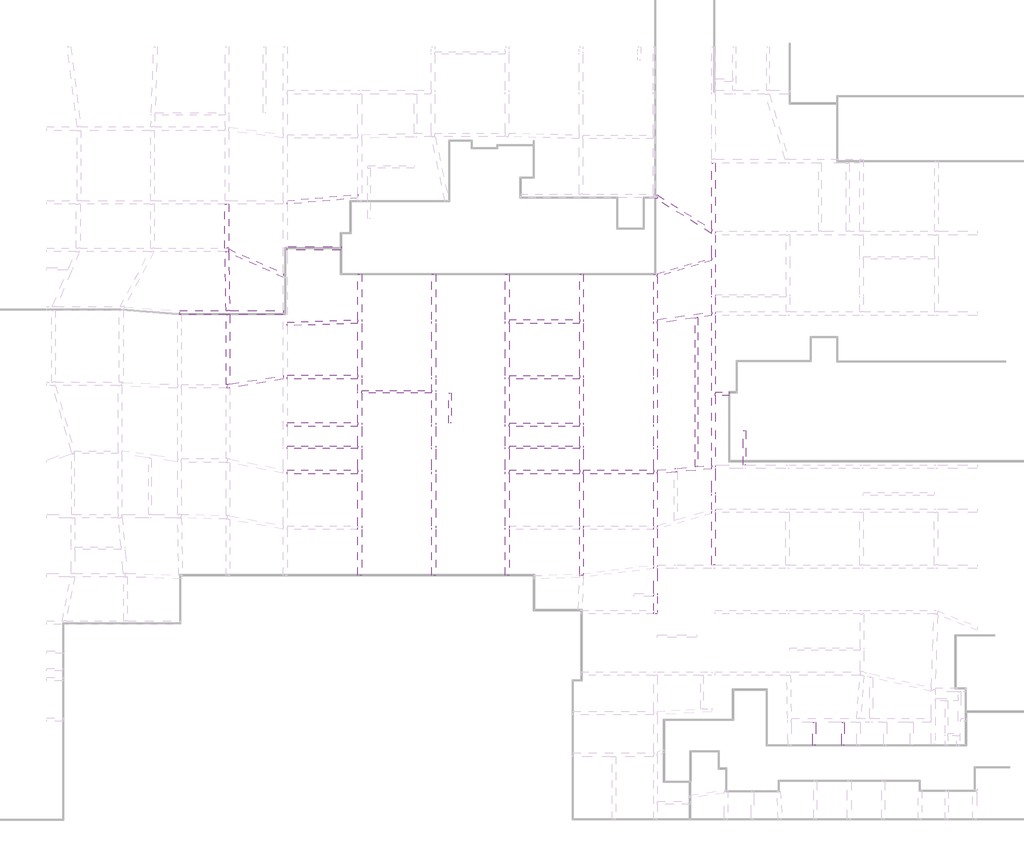
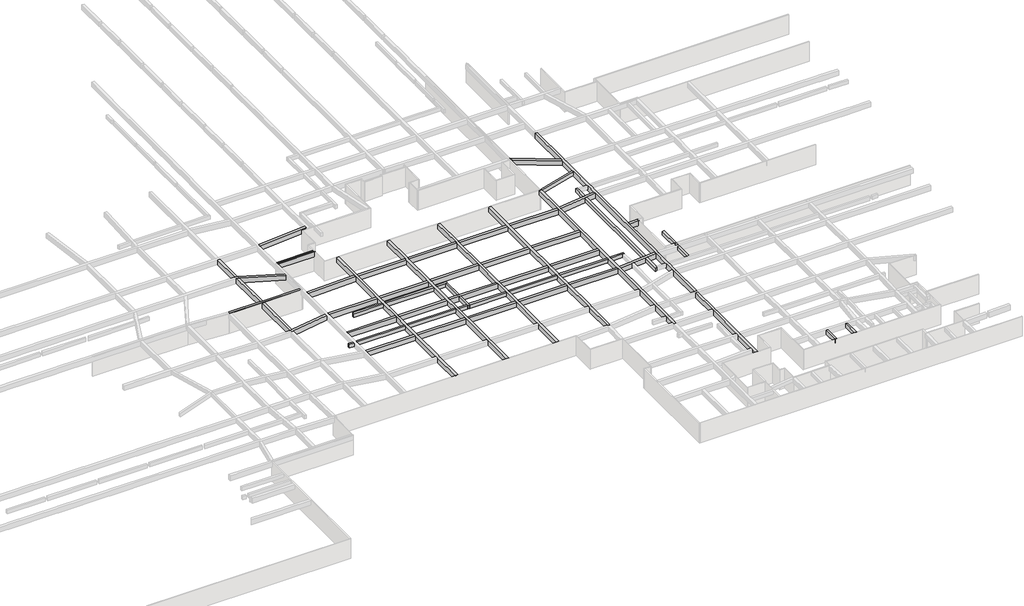
# One storey, part 9 of 16: 36 beams.
"""IFC4 building model written with IfcOpenShell, lengths in millimetres."""

from ifc_helpers import new_model, si_unit, frame, origin, place, context, project, spatial, polyline, outline, extrude, faceted_brep, element, save

model = new_model("IFC4")

# Units and contexts
model_context = context("Model", 3, world=origin())
ifc_project = project(units=[si_unit("LENGTHUNIT", "METRE", prefix="MILLI")], contexts=[model_context])

# Site, building, storey
site = spatial("IfcSite", under=ifc_project)
building = spatial("IfcBuilding", under=site)
storey = spatial("IfcBuildingStorey", under=building, Name="户型图", Elevation=0.0)

# Beams
placement = place(None, origin())
element("IfcBeam", 1, ObjectType="混凝土 - 矩形梁 : KL_beam", at=placement, inside=storey, context=model_context, shape_type="Brep", body=[
    faceted_brep([(188116.2109037, 124102.5628076, 3300.0), (188116.2109037, 124574.2341689, 3300.0), (182116.2109037, 128323.4502804, 3300.0), (182116.2109037, 128212.6640931, 3300.0), (182116.2109037, 128072.5884701, 3300.0), (182216.2109037, 128072.5884701, 3300.0), (182216.2109037, 127952.5884701, 3300.0), (181954.8818982, 127952.5884701, 3300.0), (188116.2109037, 124102.5628076, 2500.0), (181954.8818982, 127952.5884701, 2500.0), (188116.2109037, 124574.2341689, 2500.0), (182216.2109037, 127952.5884701, 2500.0), (182216.2109037, 128072.5884701, 2500.0), (182116.2109037, 128072.5884701, 2500.0), (182116.2109037, 128212.6640931, 2500.0), (182116.2109037, 128323.4502804, 2500.0)], [[[0, 1, 2, 3, 4, 5, 6, 7]], [[8, 0, 7, 9]], [[10, 8, 9, 11, 12, 13, 14, 15]], [[15, 2, 1, 10]], [[2, 15, 14, 13, 4, 3]], [[1, 0, 8, 10]], [[6, 11, 9, 7]], [[12, 5, 4, 13]], [[11, 6, 5, 12]]]),
])
element("IfcBeam", 2, ObjectType="混凝土 - 矩形梁 : KL_beam", at=placement, inside=storey, context=model_context, shape_type="Brep", body=[
    faceted_brep([(149816.2109037, 86683.8704175, 3300.0), (149416.2109037, 86683.8704175, 3300.0), (149416.2109037, 86683.8704175, 2500.0), (149816.2109037, 86683.8704175, 2500.0), (149816.2109037, 119637.8704175, 3300.0), (149816.2109037, 119637.8704175, 2500.0), (149416.2109037, 119637.8704175, 2500.0), (149416.2109037, 119637.8704175, 3300.0), (149816.2109037, 91682.2447201, 3300.0), (149816.2109037, 92082.2447201, 3300.0), (149816.2109037, 97782.2759701, 3300.0), (149816.2109037, 98182.2759701, 3300.0), (149816.2109037, 100527.3152457, 3300.0), (149816.2109037, 100827.3152457, 3300.0), (149816.2109037, 102960.8704175, 3300.0), (149816.2109037, 103360.8704175, 3300.0), (149816.2109037, 106627.3152457, 3300.0), (149816.2109037, 106927.3152457, 3300.0), (149816.2109037, 108132.2759701, 3300.0), (149816.2109037, 108532.2759701, 3300.0), (149816.2109037, 114242.5776022, 3300.0), (149816.2109037, 114642.5776022, 3300.0), (149416.2109037, 114636.4344095, 3300.0), (149416.2109037, 114236.2397358, 3300.0), (149416.2109037, 108582.2759701, 3300.0), (149416.2109037, 108182.2759701, 3300.0), (149416.2109037, 106927.3152457, 3300.0), (149416.2109037, 106627.3152457, 3300.0), (149416.2109037, 103382.2759701, 3300.0), (149416.2109037, 102982.2759701, 3300.0), (149416.2109037, 100827.3152457, 3300.0), (149416.2109037, 100527.3152457, 3300.0), (149416.2109037, 98182.2759701, 3300.0), (149416.2109037, 97782.2759701, 3300.0), (149416.2109037, 92082.2447201, 3300.0), (149416.2109037, 91682.2447201, 3300.0), (149416.2109037, 114636.4344095, 2500.0), (149416.2109037, 114236.2397358, 2500.0), (149416.2109037, 108582.2759701, 2500.0), (149416.2109037, 108182.2759701, 2500.0), (149416.2109037, 103382.2759701, 2500.0), (149416.2109037, 102982.2759701, 2500.0), (149416.2109037, 98182.2759701, 2500.0), (149416.2109037, 97782.2759701, 2500.0), (149416.2109037, 92082.2447201, 2500.0), (149416.2109037, 91682.2447201, 2500.0), (149816.2109037, 114642.5776022, 2500.0), (149816.2109037, 114242.5776022, 2500.0), (149816.2109037, 108532.2759701, 2500.0), (149816.2109037, 108132.2759701, 2500.0), (149816.2109037, 103360.8704175, 2500.0), (149816.2109037, 102960.8704175, 2500.0), (149816.2109037, 98182.2759701, 2500.0), (149816.2109037, 97782.2759701, 2500.0), (149816.2109037, 92082.2447201, 2500.0), (149816.2109037, 91682.2447201, 2500.0)], [[[0, 1, 2, 3]], [[4, 5, 6, 7]], [[1, 0, 8, 9, 10, 11, 12, 13, 14, 15, 16, 17, 18, 19, 20, 21, 4, 7, 22, 23, 24, 25, 26, 27, 28, 29, 30, 31, 32, 33, 34, 35]], [[2, 1, 35, 34, 33, 32, 31, 30, 29, 28, 27, 26, 25, 24, 23, 22, 7, 6, 36, 37, 38, 39, 40, 41, 42, 43, 44, 45]], [[3, 2, 45, 44, 43, 42, 41, 40, 39, 38, 37, 36, 6, 5, 46, 47, 48, 49, 50, 51, 52, 53, 54, 55]], [[0, 3, 55, 54, 53, 52, 51, 50, 49, 48, 47, 46, 5, 4, 21, 20, 19, 18, 17, 16, 15, 14, 13, 12, 11, 10, 9, 8]]]),
])
element("IfcBeam", 3, ObjectType="混凝土 - 矩形梁 : KL_beam", at=placement, inside=storey, context=model_context, shape_type="Brep", body=[
    faceted_brep([(157903.2890287, 86683.8704175, 3300.0), (157503.2890287, 86683.8704175, 3300.0), (157503.2890287, 86683.8704175, 2500.0), (157903.2890287, 86683.8704175, 2500.0), (157903.2890287, 119637.8704175, 3300.0), (157903.2890287, 119637.8704175, 2500.0), (157503.2890287, 119637.8704175, 2500.0), (157503.2890287, 119637.8704175, 3300.0), (157903.2890287, 91682.2447201, 3300.0), (157903.2890287, 92082.2447201, 3300.0), (157903.2890287, 97782.2759701, 3300.0), (157903.2890287, 98182.2759701, 3300.0), (157903.2890287, 100527.3152457, 3300.0), (157903.2890287, 100827.3152457, 3300.0), (157903.2890287, 102960.8704175, 3300.0), (157903.2890287, 103360.8704175, 3300.0), (157903.2890287, 106627.3152457, 3300.0), (157903.2890287, 106927.3152457, 3300.0), (157903.2890287, 108132.2759701, 3300.0), (157903.2890287, 108532.2759701, 3300.0), (157903.2890287, 114242.5776022, 3300.0), (157903.2890287, 114642.5776022, 3300.0), (157503.2890287, 114642.5776022, 3300.0), (157503.2890287, 114242.5776022, 3300.0), (157503.2890287, 108532.2759701, 3300.0), (157503.2890287, 108132.2759701, 3300.0), (157503.2890287, 106927.3152457, 3300.0), (157503.2890287, 106627.3152457, 3300.0), (157503.2890287, 103360.8704175, 3300.0), (157503.2890287, 102960.8704175, 3300.0), (157503.2890287, 100827.3152457, 3300.0), (157503.2890287, 100527.3152457, 3300.0), (157503.2890287, 98182.2759701, 3300.0), (157503.2890287, 97782.2759701, 3300.0), (157503.2890287, 92082.2447201, 3300.0), (157503.2890287, 91682.2447201, 3300.0), (157503.2890287, 114642.5776022, 2500.0), (157503.2890287, 114242.5776022, 2500.0), (157503.2890287, 108532.2759701, 2500.0), (157503.2890287, 108132.2759701, 2500.0), (157503.2890287, 103360.8704175, 2500.0), (157503.2890287, 102960.8704175, 2500.0), (157503.2890287, 98182.2759701, 2500.0), (157503.2890287, 97782.2759701, 2500.0), (157503.2890287, 92082.2447201, 2500.0), (157503.2890287, 91682.2447201, 2500.0), (157903.2890287, 114642.5776022, 2500.0), (157903.2890287, 114242.5776022, 2500.0), (157903.2890287, 108532.2759701, 2500.0), (157903.2890287, 108132.2759701, 2500.0), (157903.2890287, 103360.8704175, 2500.0), (157903.2890287, 102960.8704175, 2500.0), (157903.2890287, 98182.2759701, 2500.0), (157903.2890287, 97782.2759701, 2500.0), (157903.2890287, 92082.2447201, 2500.0), (157903.2890287, 91682.2447201, 2500.0)], [[[0, 1, 2, 3]], [[4, 5, 6, 7]], [[1, 0, 8, 9, 10, 11, 12, 13, 14, 15, 16, 17, 18, 19, 20, 21, 4, 7, 22, 23, 24, 25, 26, 27, 28, 29, 30, 31, 32, 33, 34, 35]], [[2, 1, 35, 34, 33, 32, 31, 30, 29, 28, 27, 26, 25, 24, 23, 22, 7, 6, 36, 37, 38, 39, 40, 41, 42, 43, 44, 45]], [[3, 2, 45, 44, 43, 42, 41, 40, 39, 38, 37, 36, 6, 5, 46, 47, 48, 49, 50, 51, 52, 53, 54, 55]], [[0, 3, 55, 54, 53, 52, 51, 50, 49, 48, 47, 46, 5, 4, 21, 20, 19, 18, 17, 16, 15, 14, 13, 12, 11, 10, 9, 8]]]),
])
element("IfcBeam", 4, ObjectType="混凝土 - 矩形梁 : KL_beam", at=placement, inside=storey, context=model_context, shape_type="Brep", body=[
    faceted_brep([(165953.2890287, 86683.8704175, 3300.0), (165553.2890287, 86683.8704175, 3300.0), (165553.2890287, 86683.8704175, 2500.0), (165953.2890287, 86683.8704175, 2500.0), (165953.2890287, 119637.8704175, 3300.0), (165953.2890287, 119637.8704175, 2500.0), (165553.2890287, 119637.8704175, 2500.0), (165553.2890287, 119637.8704175, 3300.0), (165953.2890287, 91682.2447201, 3300.0), (165953.2890287, 92082.2447201, 3300.0), (165953.2890287, 97782.2759701, 3300.0), (165953.2890287, 98182.2759701, 3300.0), (165953.2890287, 100527.3152457, 3300.0), (165953.2890287, 100827.3152457, 3300.0), (165953.2890287, 102960.8704175, 3300.0), (165953.2890287, 103360.8704175, 3300.0), (165953.2890287, 108132.2759701, 3300.0), (165953.2890287, 108532.2759701, 3300.0), (165953.2890287, 114242.5776022, 3300.0), (165953.2890287, 114642.5776022, 3300.0), (165553.2890287, 114642.5776022, 3300.0), (165553.2890287, 114242.5776022, 3300.0), (165553.2890287, 108532.2759701, 3300.0), (165553.2890287, 108132.2759701, 3300.0), (165553.2890287, 103360.8704175, 3300.0), (165553.2890287, 102960.8704175, 3300.0), (165553.2890287, 100827.3152457, 3300.0), (165553.2890287, 100527.3152457, 3300.0), (165553.2890287, 98182.2759701, 3300.0), (165553.2890287, 97782.2759701, 3300.0), (165553.2890287, 92082.2447201, 3300.0), (165553.2890287, 91682.2447201, 3300.0), (165553.2890287, 114642.5776022, 2500.0), (165553.2890287, 114242.5776022, 2500.0), (165553.2890287, 108532.2759701, 2500.0), (165553.2890287, 108132.2759701, 2500.0), (165553.2890287, 103360.8704175, 2500.0), (165553.2890287, 102960.8704175, 2500.0), (165553.2890287, 98182.2759701, 2500.0), (165553.2890287, 97782.2759701, 2500.0), (165553.2890287, 92082.2447201, 2500.0), (165553.2890287, 91682.2447201, 2500.0), (165953.2890287, 114642.5776022, 2500.0), (165953.2890287, 114242.5776022, 2500.0), (165953.2890287, 108532.2759701, 2500.0), (165953.2890287, 108132.2759701, 2500.0), (165953.2890287, 103360.8704175, 2500.0), (165953.2890287, 102960.8704175, 2500.0), (165953.2890287, 98182.2759701, 2500.0), (165953.2890287, 97782.2759701, 2500.0), (165953.2890287, 92082.2447201, 2500.0), (165953.2890287, 91682.2447201, 2500.0)], [[[0, 1, 2, 3]], [[4, 5, 6, 7]], [[1, 0, 8, 9, 10, 11, 12, 13, 14, 15, 16, 17, 18, 19, 4, 7, 20, 21, 22, 23, 24, 25, 26, 27, 28, 29, 30, 31]], [[2, 1, 31, 30, 29, 28, 27, 26, 25, 24, 23, 22, 21, 20, 7, 6, 32, 33, 34, 35, 36, 37, 38, 39, 40, 41]], [[3, 2, 41, 40, 39, 38, 37, 36, 35, 34, 33, 32, 6, 5, 42, 43, 44, 45, 46, 47, 48, 49, 50, 51]], [[0, 3, 51, 50, 49, 48, 47, 46, 45, 44, 43, 42, 5, 4, 19, 18, 17, 16, 15, 14, 13, 12, 11, 10, 9, 8]]]),
])
element("IfcBeam", 5, ObjectType="混凝土 - 矩形梁 : KL_beam", at=placement, inside=storey, context=model_context, shape_type="Brep", body=[
    faceted_brep([(174063.2890287, 119638.0279232, 3300.0), (174063.2890287, 119638.0279232, 2500.0), (173663.2890287, 119638.0279232, 2500.0), (173663.2890287, 119638.0279232, 3300.0), (173663.2890287, 86641.5189362, 3300.0), (174063.2890287, 86634.5369102, 3300.0), (174063.2890287, 86864.0868005, 3300.0), (174063.2890287, 91682.2447201, 3300.0), (174063.2890287, 92082.2447201, 3300.0), (174063.2890287, 97782.2759701, 3300.0), (174063.2890287, 98182.2759701, 3300.0), (174063.2890287, 100527.3152457, 3300.0), (174063.2890287, 100827.3152457, 3300.0), (174063.2890287, 102960.8704175, 3300.0), (174063.2890287, 103360.8704175, 3300.0), (174063.2890287, 108132.2759701, 3300.0), (174063.2890287, 108532.2759701, 3300.0), (174063.2890287, 114242.5776022, 3300.0), (174063.2890287, 114642.5776022, 3300.0), (173663.2890287, 114642.5776022, 3300.0), (173663.2890287, 114242.5776022, 3300.0), (173663.2890287, 108532.2759701, 3300.0), (173663.2890287, 108132.2759701, 3300.0), (173663.2890287, 103360.8704175, 3300.0), (173663.2890287, 102960.8704175, 3300.0), (173663.2890287, 100827.3152457, 3300.0), (173663.2890287, 100527.3152457, 3300.0), (173663.2890287, 98182.2759701, 3300.0), (173663.2890287, 97782.2759701, 3300.0), (173663.2890287, 92082.2447201, 3300.0), (173663.2890287, 91682.2447201, 3300.0), (173663.2890287, 86831.1656782, 3300.0), (173663.2890287, 86641.5189362, 2500.0), (173663.2890287, 114642.5776022, 2500.0), (173663.2890287, 114242.5776022, 2500.0), (173663.2890287, 108532.2759701, 2500.0), (173663.2890287, 108132.2759701, 2500.0), (173663.2890287, 103360.8704175, 2500.0), (173663.2890287, 102960.8704175, 2500.0), (173663.2890287, 98182.2759701, 2500.0), (173663.2890287, 97782.2759701, 2500.0), (173663.2890287, 92082.2447201, 2500.0), (173663.2890287, 91682.2447201, 2500.0), (173663.2890287, 86831.1656782, 2500.0), (174063.2890287, 86634.5369102, 2500.0), (174063.2890287, 114642.5776022, 2500.0), (174063.2890287, 114242.5776022, 2500.0), (174063.2890287, 108532.2759701, 2500.0), (174063.2890287, 108132.2759701, 2500.0), (174063.2890287, 103360.8704175, 2500.0), (174063.2890287, 102960.8704175, 2500.0), (174063.2890287, 98182.2759701, 2500.0), (174063.2890287, 97782.2759701, 2500.0), (174063.2890287, 92082.2447201, 2500.0), (174063.2890287, 91682.2447201, 2500.0), (174063.2890287, 86864.0868005, 2500.0)], [[[0, 1, 2, 3]], [[4, 5, 6, 7, 8, 9, 10, 11, 12, 13, 14, 15, 16, 17, 18, 0, 3, 19, 20, 21, 22, 23, 24, 25, 26, 27, 28, 29, 30, 31]], [[32, 4, 31, 30, 29, 28, 27, 26, 25, 24, 23, 22, 21, 20, 19, 3, 2, 33, 34, 35, 36, 37, 38, 39, 40, 41, 42, 43]], [[44, 32, 43, 42, 41, 40, 39, 38, 37, 36, 35, 34, 33, 2, 1, 45, 46, 47, 48, 49, 50, 51, 52, 53, 54, 55]], [[5, 44, 55, 54, 53, 52, 51, 50, 49, 48, 47, 46, 45, 1, 0, 18, 17, 16, 15, 14, 13, 12, 11, 10, 9, 8, 7, 6]], [[5, 4, 32, 44]]]),
])
element("IfcBeam", 6, ObjectType="混凝土 - 矩形梁 : KL_beam", at=placement, inside=storey, context=model_context, shape_type="SweptSolid", body=[
    extrude(outline(polyline([(149816.2109037, 114242.5776022), (149816.2109037, 114642.5776022), (157503.2890287, 114642.5776022), (157503.2890287, 114242.5776022), (149816.2109037, 114242.5776022)])), frame((0.0, 0.0, 2500.0), z_axis=(0.0, 0.0, 1.0), x_axis=(1.0, 0.0, 0.0)), (0.0, 0.0, 1.0), 800.0),
    extrude(outline(polyline([(157903.2890287, 114242.5776022), (157903.2890287, 114642.5776022), (165553.2890287, 114642.5776022), (165553.2890287, 114242.5776022), (157903.2890287, 114242.5776022)])), frame((0.0, 0.0, 2500.0), z_axis=(0.0, 0.0, 1.0), x_axis=(1.0, 0.0, 0.0)), (0.0, 0.0, 1.0), 800.0),
    extrude(outline(polyline([(165953.2890287, 114242.5776022), (165953.2890287, 114642.5776022), (173663.2890287, 114642.5776022), (173663.2890287, 114242.5776022), (165953.2890287, 114242.5776022)])), frame((0.0, 0.0, 2500.0), z_axis=(0.0, 0.0, 1.0), x_axis=(1.0, 0.0, 0.0)), (0.0, 0.0, 1.0), 800.0),
    extrude(outline(polyline([(174063.2890287, 114242.5776022), (174063.2890287, 114642.5776022), (181757.7367524, 114642.5776022), (181757.7367524, 114242.5776022), (174063.2890287, 114242.5776022)])), frame((0.0, 0.0, 2500.0), z_axis=(0.0, 0.0, 1.0), x_axis=(1.0, 0.0, 0.0)), (0.0, 0.0, 1.0), 800.0),
])
element("IfcBeam", 7, ObjectType="混凝土 - 矩形梁 : KL_beam", at=placement, inside=storey, context=model_context, shape_type="SweptSolid", body=[
    extrude(outline(polyline([(149816.2109037, 108132.2759701), (149816.2109037, 108532.2759701), (157503.2890287, 108532.2759701), (157503.2890287, 108132.2759701), (149816.2109037, 108132.2759701)])), frame((0.0, 0.0, 2500.0), z_axis=(0.0, 0.0, 1.0), x_axis=(1.0, 0.0, 0.0)), (0.0, 0.0, 1.0), 800.0),
    extrude(outline(polyline([(157903.2890287, 108132.2759701), (157903.2890287, 108532.2759701), (165553.2890287, 108532.2759701), (165553.2890287, 108132.2759701), (157903.2890287, 108132.2759701)])), frame((0.0, 0.0, 2500.0), z_axis=(0.0, 0.0, 1.0), x_axis=(1.0, 0.0, 0.0)), (0.0, 0.0, 1.0), 800.0),
    extrude(outline(polyline([(165953.2890287, 108132.2759701), (165953.2890287, 108532.2759701), (173663.2890287, 108532.2759701), (173663.2890287, 108132.2759701), (165953.2890287, 108132.2759701)])), frame((0.0, 0.0, 2500.0), z_axis=(0.0, 0.0, 1.0), x_axis=(1.0, 0.0, 0.0)), (0.0, 0.0, 1.0), 800.0),
    extrude(outline(polyline([(174063.2890287, 108132.2759701), (174063.2890287, 108532.2759701), (181757.7367524, 108532.2759701), (181757.7367524, 108132.2759701), (174063.2890287, 108132.2759701)])), frame((0.0, 0.0, 2500.0), z_axis=(0.0, 0.0, 1.0), x_axis=(1.0, 0.0, 0.0)), (0.0, 0.0, 1.0), 800.0),
])
element("IfcBeam", 8, ObjectType="混凝土 - 矩形梁 : KL_beam", at=placement, inside=storey, context=model_context, shape_type="Brep", body=[
    faceted_brep([(149816.2109037, 103360.8704175, 3300.0), (149816.2109037, 102960.8704175, 3300.0), (157503.2890287, 102960.8704175, 3300.0), (157503.2890287, 103360.8704175, 3300.0), (149816.2109037, 102960.8704175, 2500.0), (157503.2890287, 102960.8704175, 2500.0), (149816.2109037, 103360.8704175, 2500.0), (157503.2890287, 103360.8704175, 2500.0)], [[[0, 1, 2, 3]], [[1, 4, 5, 2]], [[4, 6, 7, 5]], [[6, 0, 3, 7]], [[1, 0, 6, 4]], [[3, 2, 5, 7]]]),
    faceted_brep([(157903.2890287, 102960.8704175, 3300.0), (157903.2890287, 103360.8704175, 3300.0), (157903.2890287, 103360.8704175, 2500.0), (157903.2890287, 102960.8704175, 2500.0), (165553.2890287, 103360.8704175, 3300.0), (165553.2890287, 102960.8704175, 3300.0), (165553.2890287, 102960.8704175, 2500.0), (165553.2890287, 103360.8704175, 2500.0), (159337.9237533, 102960.8704175, 3300.0), (159637.9237533, 102960.8704175, 3300.0), (159637.9237533, 103360.8704175, 3300.0), (159337.9237533, 103360.8704175, 3300.0)], [[[0, 1, 2, 3]], [[4, 5, 6, 7]], [[1, 0, 8, 9, 5, 4, 10, 11]], [[0, 3, 6, 5, 9, 8]], [[3, 2, 7, 6]], [[2, 1, 11, 10, 4, 7]]]),
    faceted_brep([(165953.2890287, 103360.8704175, 3300.0), (165953.2890287, 102960.8704175, 3300.0), (173663.2890287, 102960.8704175, 3300.0), (173663.2890287, 103360.8704175, 3300.0), (165953.2890287, 102960.8704175, 2500.0), (173663.2890287, 102960.8704175, 2500.0), (165953.2890287, 103360.8704175, 2500.0), (173663.2890287, 103360.8704175, 2500.0)], [[[0, 1, 2, 3]], [[1, 4, 5, 2]], [[4, 6, 7, 5]], [[6, 0, 3, 7]], [[1, 0, 6, 4]], [[3, 2, 5, 7]]]),
    faceted_brep([(174063.2890287, 102960.8704175, 3300.0), (174063.2890287, 103360.8704175, 3300.0), (174063.2890287, 103360.8704175, 2500.0), (174063.2890287, 102960.8704175, 2500.0), (181757.7367524, 102960.8704175, 3300.0), (181757.7367524, 103360.8704175, 3300.0), (181757.7367524, 102960.8704175, 2500.0), (181757.7367524, 103360.8704175, 2500.0)], [[[0, 1, 2, 3]], [[1, 0, 4, 5]], [[0, 3, 6, 4]], [[3, 2, 7, 6]], [[2, 1, 5, 7]], [[5, 4, 6, 7]]]),
])
element("IfcBeam", 9, ObjectType="混凝土 - 矩形梁 : KL_beam", at=placement, inside=storey, context=model_context, shape_type="SweptSolid", body=[
    extrude(outline(polyline([(149816.2109037, 97782.2759701), (149816.2109037, 98182.2759701), (157503.2890287, 98182.2759701), (157503.2890287, 97782.2759701), (149816.2109037, 97782.2759701)])), frame((0.0, 0.0, 2500.0), z_axis=(0.0, 0.0, 1.0), x_axis=(1.0, 0.0, 0.0)), (0.0, 0.0, 1.0), 800.0),
    extrude(outline(polyline([(173663.2890287, 98182.2759701), (173663.2890287, 97782.2759701), (165953.2890287, 97782.2759701), (165953.2890287, 98182.2759701), (173663.2890287, 98182.2759701)])), frame((0.0, 0.0, 2500.0), z_axis=(0.0, 0.0, 1.0), x_axis=(1.0, 0.0, 0.0)), (0.0, 0.0, 1.0), 800.0),
    extrude(outline(polyline([(157903.2890287, 97782.2759701), (157903.2890287, 98182.2759701), (165553.2890287, 98182.2759701), (165553.2890287, 97782.2759701), (157903.2890287, 97782.2759701)])), frame((0.0, 0.0, 2500.0), z_axis=(0.0, 0.0, 1.0), x_axis=(1.0, 0.0, 0.0)), (0.0, 0.0, 1.0), 800.0),
])
element("IfcBeam", 10, ObjectType="混凝土 - 矩形梁 : KL_beam", at=placement, inside=storey, context=model_context, shape_type="SweptSolid", body=[
    extrude(outline(polyline([(141666.2091209, 113994.4191627), (141666.2091209, 114394.6138364), (149416.2109037, 114636.4344095), (149416.2109037, 114236.2397358), (141666.2091209, 113994.4191627)])), frame((0.0, 0.0, 2500.0), z_axis=(0.0, 0.0, 1.0), x_axis=(1.0, 0.0, 0.0)), (0.0, 0.0, 1.0), 800.0),
])
element("IfcBeam", 11, ObjectType="混凝土 - 矩形梁 : KL_beam", at=placement, inside=storey, context=model_context, shape_type="SweptSolid", body=[
    extrude(outline(polyline([(141666.2091209, 108182.2759701), (141666.2091209, 108582.2759701), (149416.2109037, 108582.2759701), (149416.2109037, 108182.2759701), (141666.2091209, 108182.2759701)])), frame((0.0, 0.0, 2500.0), z_axis=(0.0, 0.0, 1.0), x_axis=(1.0, 0.0, 0.0)), (0.0, 0.0, 1.0), 800.0),
])
element("IfcBeam", 12, ObjectType="混凝土 - 矩形梁 : KL_beam", at=placement, inside=storey, context=model_context, shape_type="SweptSolid", body=[
    extrude(outline(polyline([(141666.2091209, 102982.2759701), (141666.2091209, 103382.2759701), (149416.2109037, 103382.2759701), (149416.2109037, 102982.2759701), (141666.2091209, 102982.2759701)])), frame((0.0, 0.0, 2500.0), z_axis=(0.0, 0.0, 1.0), x_axis=(1.0, 0.0, 0.0)), (0.0, 0.0, 1.0), 800.0),
])
element("IfcBeam", 13, ObjectType="混凝土 - 矩形梁 : KL_beam", at=placement, inside=storey, context=model_context, shape_type="SweptSolid", body=[
    extrude(outline(polyline([(141666.2091209, 97782.2759701), (141666.2091209, 98182.2759701), (149416.2109037, 98182.2759701), (149416.2109037, 97782.2759701), (141666.2091209, 97782.2759701)])), frame((0.0, 0.0, 2500.0), z_axis=(0.0, 0.0, 1.0), x_axis=(1.0, 0.0, 0.0)), (0.0, 0.0, 1.0), 800.0),
])
element("IfcBeam", 14, ObjectType="混凝土 - 矩形梁 : KL_beam", at=placement, inside=storey, context=model_context, shape_type="SweptSolid", body=[
    extrude(outline(polyline([(141666.2091209, 127294.7597353), (141666.2091209, 127696.2876703), (149416.2109037, 128374.3249686), (149416.2109037, 127972.7970336), (141666.2091209, 127294.7597353)])), frame((0.0, 0.0, 2500.0), z_axis=(0.0, 0.0, 1.0), x_axis=(1.0, 0.0, 0.0)), (0.0, 0.0, 1.0), 800.0),
])
element("IfcBeam", 15, ObjectType="混凝土 - 矩形梁 : KL_beam", at=placement, inside=storey, context=model_context, shape_type="Brep", body=[
    faceted_brep([(129907.8578626, 115630.3247929, 3300.0), (129893.8895548, 115230.3247929, 3300.0), (130100.8737087, 115230.3247929, 3300.0), (134985.8688171, 115230.3247929, 3300.0), (135385.8688171, 115230.3247929, 3300.0), (141266.2091209, 115230.3247929, 3300.0), (141266.2091209, 115630.3247929, 3300.0), (135382.4082697, 115630.3247929, 3300.0), (134982.3473385, 115630.3247929, 3300.0), (129893.8895548, 115230.3247929, 2500.0), (130100.8737087, 115230.3247929, 2500.0), (134985.8688171, 115230.3247929, 2500.0), (135385.8688171, 115230.3247929, 2500.0), (141266.2091209, 115230.3247929, 2500.0), (129907.8578626, 115630.3247929, 2500.0), (134982.3473385, 115630.3247929, 2500.0), (135382.4082697, 115630.3247929, 2500.0), (141266.2091209, 115630.3247929, 2500.0)], [[[0, 1, 2, 3, 4, 5, 6, 7, 8]], [[1, 9, 10, 11, 12, 13, 5, 4, 3, 2]], [[9, 14, 15, 16, 17, 13, 12, 11, 10]], [[14, 0, 8, 7, 6, 17, 16, 15]], [[0, 14, 9, 1]], [[6, 5, 13, 17]]]),
])
element("IfcBeam", 16, ObjectType="混凝土 - 矩形梁 : KL_beam", at=placement, inside=storey, context=model_context, shape_type="SweptSolid", body=[
    extrude(outline(polyline([(135266.2109037, 122485.5220623), (134866.2109037, 122485.5220623), (134866.2109037, 127293.5189202), (135266.2109037, 127293.5189202), (135266.2109037, 122485.5220623)])), frame((0.0, 0.0, 2500.0), z_axis=(0.0, 0.0, 1.0), x_axis=(1.0, 0.0, 0.0)), (0.0, 0.0, 1.0), 800.0),
])
element("IfcBeam", 17, ObjectType="混凝土 - 矩形梁 : KL_beam", at=placement, inside=storey, context=model_context, shape_type="Brep", body=[
    faceted_brep([(135266.2109037, 122085.5220623, 3300.0), (134869.671451, 122085.5220623, 3300.0), (134982.3473385, 115630.3247929, 3300.0), (135382.4082697, 115630.3247929, 3300.0), (135271.6779225, 121974.0621338, 3300.0), (135266.2109037, 122287.2674359, 3300.0), (134869.671451, 122085.5220623, 2500.0), (134982.3473385, 115630.3247929, 2500.0), (135266.2109037, 122085.5220623, 2500.0), (135266.2109037, 122287.2674359, 2500.0), (135271.6779225, 121974.0621338, 2500.0), (135382.4082697, 115630.3247929, 2500.0)], [[[0, 1, 2, 3, 4, 5]], [[1, 6, 7, 2]], [[6, 8, 9, 10, 11, 7]], [[9, 5, 4, 3, 11, 10]], [[0, 8, 6, 1]], [[8, 0, 5, 9]], [[3, 2, 7, 11]]]),
])
element("IfcBeam", 18, ObjectType="混凝土 - 矩形梁 : KL_beam", at=placement, inside=storey, context=model_context, shape_type="SweptSolid", body=[
    extrude(outline(polyline([(141266.2091209, 119721.5942757), (141266.2091209, 119283.141064), (135271.6779225, 121974.0621338), (135266.2109037, 122287.2674359), (135266.2109037, 122414.9694684), (141266.2091209, 119721.5942757)])), frame((0.0, 0.0, 2500.0), z_axis=(0.0, 0.0, 1.0), x_axis=(1.0, 0.0, 0.0)), (0.0, 0.0, 1.0), 800.0),
])
element("IfcBeam", 19, ObjectType="混凝土 - 矩形梁 : KL_beam", at=placement, inside=storey, context=model_context, shape_type="Brep", body=[
    faceted_brep([(135100.1329465, 107552.6668763, 3300.0), (135132.3513609, 107152.6668763, 3300.0), (135385.8688171, 107193.7732127, 3300.0), (141266.2091209, 108147.2351571, 3300.0), (141266.2091209, 108552.4591799, 3300.0), (135385.8688171, 107598.9972356, 3300.0), (135132.3513609, 107152.6668763, 2500.0), (135385.8688171, 107193.7732127, 2500.0), (141266.2091209, 108147.2351571, 2500.0), (135100.1329465, 107552.6668763, 2500.0), (135385.8688171, 107598.9972356, 2500.0), (141266.2091209, 108552.4591799, 2500.0)], [[[0, 1, 2, 3, 4, 5]], [[1, 6, 7, 8, 3, 2]], [[6, 9, 10, 11, 8, 7]], [[9, 0, 5, 4, 11, 10]], [[0, 9, 6, 1]], [[4, 3, 8, 11]]]),
])
element("IfcBeam", 20, ObjectType="混凝土 - 矩形梁 : KL_beam", at=placement, inside=storey, context=model_context, shape_type="SweptSolid", body=[
    extrude(outline(polyline([(147566.2091209, 122678.0259701), (147566.2091209, 122278.0259701), (141666.2091209, 122278.0259701), (141666.2091209, 122678.0259701), (147566.2091209, 122678.0259701)])), frame((0.0, 0.0, 2500.0), z_axis=(0.0, 0.0, 1.0), x_axis=(1.0, 0.0, 0.0)), (0.0, 0.0, 1.0), 800.0),
])
element("IfcBeam", 21, ObjectType="混凝土 - 矩形梁 : KL_beam", at=placement, inside=storey, context=model_context, shape_type="Brep", body=[
    faceted_brep([(181757.7367524, 82438.0259701, 3300.0), (182157.7367524, 82438.0259701, 3300.0), (182157.7367524, 82838.0259701, 3300.0), (182157.7367524, 84382.6131688, 3300.0), (182157.7367524, 84682.6131688, 3300.0), (182157.7367524, 87431.9011327, 3300.0), (182157.7367524, 87831.9011327, 3300.0), (182157.7367524, 91731.7470352, 3300.0), (182157.7367524, 92148.0295395, 3300.0), (182157.7367524, 97799.0097353, 3300.0), (182157.7367524, 98200.5376703, 3300.0), (182157.7367524, 100527.3152457, 3300.0), (182157.7367524, 100827.3152457, 3300.0), (182157.7367524, 114268.3909995, 3300.0), (182157.7367524, 114672.2163883, 3300.0), (182157.7367524, 119389.3378602, 3300.0), (182157.7367524, 119701.427691, 3300.0), (181757.7367524, 119586.7295367, 3300.0), (181757.7367524, 114642.5776022, 3300.0), (181757.7367524, 114242.5776022, 3300.0), (181757.7367524, 108532.2759701, 3300.0), (181757.7367524, 108132.2759701, 3300.0), (181757.7367524, 103360.8704175, 3300.0), (181757.7367524, 102960.8704175, 3300.0), (181757.7367524, 100827.3152457, 3300.0), (181757.7367524, 100527.3152457, 3300.0), (181757.7367524, 98182.2759701, 3300.0), (181757.7367524, 97782.2759701, 3300.0), (181757.7367524, 92082.2447201, 3300.0), (181757.7367524, 91682.2447201, 3300.0), (181757.7367524, 87808.8461856, 3300.0), (181757.7367524, 87405.8422555, 3300.0), (181757.7367524, 84682.6131688, 3300.0), (181757.7367524, 84382.6131688, 3300.0), (181757.7367524, 82838.0259701, 3300.0), (181757.7367524, 82438.0259701, 2500.0), (181757.7367524, 119586.7295367, 2500.0), (181757.7367524, 114642.5776022, 2500.0), (181757.7367524, 114242.5776022, 2500.0), (181757.7367524, 108532.2759701, 2500.0), (181757.7367524, 108132.2759701, 2500.0), (181757.7367524, 103360.8704175, 2500.0), (181757.7367524, 102960.8704175, 2500.0), (181757.7367524, 98182.2759701, 2500.0), (181757.7367524, 97782.2759701, 2500.0), (181757.7367524, 92082.2447201, 2500.0), (181757.7367524, 91682.2447201, 2500.0), (181757.7367524, 87808.8461856, 2500.0), (181757.7367524, 87405.8422555, 2500.0), (181757.7367524, 82838.0259701, 2500.0), (182157.7367524, 82438.0259701, 2500.0), (182157.7367524, 119701.427691, 2500.0), (182157.7367524, 114672.2163883, 2500.0), (182157.7367524, 114268.3909995, 2500.0), (182157.7367524, 98200.5376703, 2500.0), (182157.7367524, 97799.0097353, 2500.0), (182157.7367524, 92148.0295395, 2500.0), (182157.7367524, 91731.7470352, 2500.0), (182157.7367524, 87831.9011327, 2500.0), (182157.7367524, 87431.9011327, 2500.0), (182157.7367524, 82838.0259701, 2500.0), (182157.7367524, 119701.427691, 2700.0)], [[[0, 1, 2, 3, 4, 5, 6, 7, 8, 9, 10, 11, 12, 13, 14, 15, 16, 17, 18, 19, 20, 21, 22, 23, 24, 25, 26, 27, 28, 29, 30, 31, 32, 33, 34]], [[35, 0, 34, 33, 32, 31, 30, 29, 28, 27, 26, 25, 24, 23, 22, 21, 20, 19, 18, 17, 36, 37, 38, 39, 40, 41, 42, 43, 44, 45, 46, 47, 48, 49]], [[50, 35, 49, 48, 47, 46, 45, 44, 43, 42, 41, 40, 39, 38, 37, 36, 51, 52, 53, 54, 55, 56, 57, 58, 59, 60]], [[1, 50, 60, 59, 58, 57, 56, 55, 54, 53, 52, 51, 61, 16, 15, 14, 13, 12, 11, 10, 9, 8, 7, 6, 5, 4, 3, 2]], [[1, 0, 35, 50]], [[17, 16, 61, 51, 36]]]),
])
element("IfcBeam", 22, ObjectType="混凝土 - 矩形梁 : KL_beam", at=placement, inside=storey, context=model_context, shape_type="Brep", body=[
    faceted_brep([(182157.7367524, 114268.3909995, 3300.0), (182157.7367524, 114268.3909995, 2500.0), (188116.2109037, 115094.4170039, 2500.0), (188116.2109037, 115094.4170039, 3300.0), (186611.3422117, 114885.7963669, 3300.0), (186311.3422117, 114844.2072293, 3300.0), (182157.7367524, 114672.2163883, 3300.0), (182157.7367524, 114672.2163883, 2500.0), (188116.2109037, 115498.2423927, 2500.0), (188116.2109037, 115498.2423927, 3300.0), (186611.3422117, 115289.6217557, 3300.0), (186311.3422117, 115248.0326181, 3300.0)], [[[0, 1, 2, 3, 4, 5]], [[1, 0, 6, 7]], [[3, 2, 8, 9]], [[3, 9, 10, 11, 6, 0, 5, 4]], [[8, 2, 1, 7]], [[9, 8, 7, 6, 11, 10]]]),
])
element("IfcBeam", 23, ObjectType="混凝土 - 矩形梁 : KL_beam", at=placement, inside=storey, context=model_context, shape_type="SweptSolid", body=[
    extrude(outline(polyline([(174063.2890287, 97782.2759701), (174063.2890287, 98182.2759701), (181757.7367524, 98182.2759701), (181757.7367524, 97782.2759701), (174063.2890287, 97782.2759701)])), frame((0.0, 0.0, 2500.0), z_axis=(0.0, 0.0, 1.0), x_axis=(1.0, 0.0, 0.0)), (0.0, 0.0, 1.0), 800.0),
])
element("IfcBeam", 24, ObjectType="混凝土 - 矩形梁 : KL_beam", at=placement, inside=storey, context=model_context, shape_type="Brep", body=[
    faceted_brep([(182157.7367524, 98200.5376703, 3300.0), (182157.7367524, 97799.0097353, 3300.0), (184037.9237533, 97963.5047832, 3300.0), (184337.9237533, 97989.7513822, 3300.0), (186311.3422117, 98162.4031257, 3300.0), (186611.3422117, 98188.6497248, 3300.0), (188116.2109037, 98320.3086754, 3300.0), (188116.2109037, 98721.8366105, 3300.0), (186611.3422117, 98590.1776598, 3300.0), (186311.3422117, 98563.9310608, 3300.0), (184337.9237533, 98391.2793173, 3300.0), (184037.9237533, 98365.0327182, 3300.0), (182157.7367524, 97799.0097353, 2500.0), (188116.2109037, 98320.3086754, 2500.0), (182157.7367524, 98200.5376703, 2500.0), (188116.2109037, 98721.8366105, 2500.0)], [[[0, 1, 2, 3, 4, 5, 6, 7, 8, 9, 10, 11]], [[1, 12, 13, 6, 5, 4, 3, 2]], [[12, 14, 15, 13]], [[14, 0, 11, 10, 9, 8, 7, 15]], [[1, 0, 14, 12]], [[7, 6, 13, 15]]]),
])
element("IfcBeam", 25, ObjectType="混凝土 - 矩形梁 : KL_beam", at=placement, inside=storey, context=model_context, shape_type="Brep", body=[
    faceted_brep([(188516.2109037, 70862.3072201, 3300.0), (188116.2109037, 70862.3072201, 3300.0), (188116.2109037, 70862.3072201, 2500.0), (188516.2109037, 70862.3072201, 2500.0), (188516.2109037, 75726.6254049, 3300.0), (188516.2109037, 76126.6254049, 3300.0), (188516.2109037, 82438.0259701, 3300.0), (188516.2109037, 82838.0259701, 3300.0), (188516.2109037, 87431.9011327, 3300.0), (188116.2109037, 87431.9011327, 3300.0), (188116.2109037, 82838.0259701, 3300.0), (188116.2109037, 82438.0259701, 3300.0), (188116.2109037, 76126.6254049, 3300.0), (188116.2109037, 75726.6254049, 3300.0), (188116.2109037, 72101.9126334, 3300.0), (188116.2109037, 71701.363695, 3300.0), (188116.2109037, 87431.9011327, 2500.0), (188116.2109037, 82838.0259701, 2500.0), (188116.2109037, 82438.0259701, 2500.0), (188116.2109037, 76126.6254049, 2500.0), (188116.2109037, 75726.6254049, 2500.0), (188116.2109037, 72101.9126334, 2500.0), (188116.2109037, 71701.363695, 2500.0), (188516.2109037, 87431.9011327, 2500.0), (188516.2109037, 82838.0259701, 2500.0), (188516.2109037, 82438.0259701, 2500.0), (188516.2109037, 76126.6254049, 2500.0), (188516.2109037, 75726.6254049, 2500.0)], [[[0, 1, 2, 3]], [[1, 0, 4, 5, 6, 7, 8, 9, 10, 11, 12, 13, 14, 15]], [[2, 1, 15, 14, 13, 12, 11, 10, 9, 16, 17, 18, 19, 20, 21, 22]], [[3, 2, 22, 21, 20, 19, 18, 17, 16, 23, 24, 25, 26, 27]], [[0, 3, 27, 26, 25, 24, 23, 8, 7, 6, 5, 4]], [[9, 8, 23, 16]]]),
    faceted_brep([(188116.2109037, 131811.3072201, 3300.0), (188516.2109037, 131811.3072201, 3300.0), (188516.2109037, 131811.3072201, 2500.0), (188116.2109037, 131811.3072201, 2500.0), (188516.2109037, 87831.9011327, 3300.0), (188116.2109037, 87831.9011327, 3300.0), (188116.2109037, 87831.9011327, 2500.0), (188516.2109037, 87831.9011327, 2500.0), (188116.2109037, 124574.2341689, 3300.0), (188116.2109037, 124102.5628076, 3300.0), (188116.2109037, 121409.99266, 3300.0), (188116.2109037, 121097.9028293, 3300.0), (188116.2109037, 117415.9096032, 3300.0), (188116.2109037, 117115.9096032, 3300.0), (188116.2109037, 115498.2423927, 3300.0), (188116.2109037, 115094.4170039, 3300.0), (188116.2109037, 98721.8366105, 3300.0), (188116.2109037, 98320.3086754, 3300.0), (188116.2109037, 95715.9096032, 3300.0), (188116.2109037, 95415.9096032, 3300.0), (188116.2109037, 93865.3680672, 3300.0), (188116.2109037, 93449.0855629, 3300.0), (188516.2109037, 93528.4104182, 3300.0), (188516.2109037, 93928.4104182, 3300.0), (188516.2109037, 95415.9096032, 3300.0), (188516.2109037, 95715.9096032, 3300.0), (188516.2109037, 98340.0727237, 3300.0), (188516.2109037, 98740.0727237, 3300.0), (188516.2109037, 106351.2090896, 3300.0), (188516.2109037, 106751.2090896, 3300.0), (188516.2109037, 115130.098028, 3300.0), (188516.2109037, 115530.098028, 3300.0), (188516.2109037, 117115.9096032, 3300.0), (188516.2109037, 117415.9096032, 3300.0), (188516.2109037, 123932.2101355, 3300.0), (188516.2109037, 124332.2101355, 3300.0), (188116.2109037, 124574.2341689, 2500.0), (188116.2109037, 124102.5628076, 2500.0), (188116.2109037, 115498.2423927, 2500.0), (188116.2109037, 115094.4170039, 2500.0), (188116.2109037, 98721.8366105, 2500.0), (188116.2109037, 98320.3086754, 2500.0), (188116.2109037, 93865.3680672, 2500.0), (188116.2109037, 93449.0855629, 2500.0), (188516.2109037, 124332.2101355, 2500.0), (188516.2109037, 123932.2101355, 2500.0), (188516.2109037, 115530.098028, 2500.0), (188516.2109037, 115130.098028, 2500.0), (188516.2109037, 106751.2090896, 2500.0), (188516.2109037, 106351.2090896, 2500.0), (188516.2109037, 98740.0727237, 2500.0), (188516.2109037, 98340.0727237, 2500.0), (188516.2109037, 93928.4104182, 2500.0), (188516.2109037, 93528.4104182, 2500.0)], [[[0, 1, 2, 3]], [[4, 5, 6, 7]], [[1, 0, 8, 9, 10, 11, 12, 13, 14, 15, 16, 17, 18, 19, 20, 21, 5, 4, 22, 23, 24, 25, 26, 27, 28, 29, 30, 31, 32, 33, 34, 35]], [[0, 3, 36, 37, 38, 39, 40, 41, 42, 43, 6, 5, 21, 20, 19, 18, 17, 16, 15, 14, 13, 12, 11, 10, 9, 8]], [[3, 2, 44, 45, 46, 47, 48, 49, 50, 51, 52, 53, 7, 6, 43, 42, 41, 40, 39, 38, 37, 36]], [[2, 1, 35, 34, 33, 32, 31, 30, 29, 28, 27, 26, 25, 24, 23, 22, 4, 7, 53, 52, 51, 50, 49, 48, 47, 46, 45, 44]]]),
])
element("IfcBeam", 26, ObjectType="混凝土 - 矩形梁 : KL_beam", at=placement, inside=storey, context=model_context, shape_type="SweptSolid", body=[
    extrude(outline(polyline([(190047.5696073, 106751.2090896), (190047.5696073, 106351.2090896), (188516.2109037, 106351.2090896), (188516.2109037, 106751.2090896), (190047.5696073, 106751.2090896)])), frame((0.0, 0.0, 2500.0), z_axis=(0.0, 0.0, 1.0), x_axis=(1.0, 0.0, 0.0)), (0.0, 0.0, 1.0), 800.0),
])
element("IfcBeam", 27, ObjectType="混凝土 - 矩形梁 : KL_beam", at=placement, inside=storey, context=model_context, shape_type="SweptSolid", body=[
    extrude(outline(polyline([(134985.8688171, 115230.3247929), (135385.8688171, 115230.3247929), (135385.8688171, 107598.9972356), (135100.1329465, 107552.6668763), (134985.8688171, 107552.6668763), (134985.8688171, 115230.3247929)])), frame((0.0, 0.0, 2500.0), z_axis=(0.0, 0.0, 1.0), x_axis=(1.0, 0.0, 0.0)), (0.0, 0.0, 1.0), 800.0),
])
element("IfcBeam", 28, ObjectType="混凝土 - 矩形梁 : L_beam", at=placement, inside=storey, context=model_context, shape_type="Brep", body=[
    faceted_brep([(144723.8471253, 106927.3152457, 3300.0), (144723.8471253, 106927.3152457, 2700.0), (144723.8471253, 106627.3152457, 2700.0), (144723.8471253, 106627.3152457, 3300.0), (149416.2109037, 106927.3152457, 3300.0), (149416.2109037, 106627.3152457, 3300.0), (149416.2109037, 106627.3152457, 2700.0), (149416.2109037, 106927.3152457, 2700.0)], [[[0, 1, 2, 3]], [[4, 5, 6, 7]], [[0, 3, 5, 4]], [[3, 2, 6, 5]], [[2, 1, 7, 6]], [[1, 0, 4, 7]]]),
    faceted_brep([(149816.2109037, 106927.3152457, 3300.0), (149816.2109037, 106627.3152457, 3300.0), (157503.2890287, 106627.3152457, 3300.0), (157503.2890287, 106927.3152457, 3300.0), (149816.2109037, 106627.3152457, 2700.0), (157503.2890287, 106627.3152457, 2700.0), (149816.2109037, 106927.3152457, 2700.0), (157503.2890287, 106927.3152457, 2700.0)], [[[0, 1, 2, 3]], [[1, 4, 5, 2]], [[4, 6, 7, 5]], [[6, 0, 3, 7]], [[1, 0, 6, 4]], [[3, 2, 5, 7]]]),
    faceted_brep([(157903.2890287, 106627.3152457, 3300.0), (157903.2890287, 106927.3152457, 3300.0), (157903.2890287, 106927.3152457, 2700.0), (157903.2890287, 106627.3152457, 2700.0), (159637.9237533, 106627.3152457, 3300.0), (159637.9237533, 106927.3152457, 3300.0), (159337.9237533, 106627.3152457, 3300.0), (159637.9237533, 106627.3152457, 2700.0), (159337.9237533, 106627.3152457, 2700.0), (159637.9237533, 106927.3152457, 2700.0)], [[[0, 1, 2, 3]], [[4, 5, 1, 0, 6]], [[7, 4, 6, 0, 3, 8]], [[9, 7, 8, 3, 2]], [[5, 9, 2, 1]], [[5, 4, 7, 9]]]),
])
element("IfcBeam", 29, ObjectType="混凝土 - 矩形梁 : L_beam", at=placement, inside=storey, context=model_context, shape_type="Brep", body=[
    faceted_brep([(159637.9237533, 106627.3152457, 3300.0), (159337.9237533, 106627.3152457, 3300.0), (159337.9237533, 103360.8704175, 3300.0), (159637.9237533, 103360.8704175, 3300.0), (159337.9237533, 106627.3152457, 2700.0), (159337.9237533, 103360.8704175, 2700.0), (159637.9237533, 106627.3152457, 2700.0), (159637.9237533, 103360.8704175, 2700.0)], [[[0, 1, 2, 3]], [[1, 4, 5, 2]], [[4, 6, 7, 5]], [[6, 0, 3, 7]], [[1, 0, 6, 4]], [[3, 2, 5, 7]]]),
    faceted_brep([(159337.9237533, 102960.8704175, 3300.0), (159637.9237533, 102960.8704175, 3300.0), (159637.9237533, 102960.8704175, 2700.0), (159337.9237533, 102960.8704175, 2700.0), (159337.9237533, 100527.3152457, 3300.0), (159637.9237533, 100527.3152457, 3300.0), (159637.9237533, 100827.3152457, 3300.0), (159337.9237533, 100827.3152457, 3300.0), (159337.9237533, 100527.3152457, 2700.0), (159337.9237533, 100827.3152457, 2700.0), (159637.9237533, 100527.3152457, 2700.0), (159637.9237533, 100827.3152457, 2700.0)], [[[0, 1, 2, 3]], [[4, 5, 6, 1, 0, 7]], [[8, 4, 7, 0, 3, 9]], [[10, 8, 9, 3, 2, 11]], [[5, 10, 11, 2, 1, 6]], [[5, 4, 8, 10]]]),
])
element("IfcBeam", 30, ObjectType="混凝土 - 矩形梁 : L_beam", at=placement, inside=storey, context=model_context, shape_type="Brep", body=[
    faceted_brep([(159637.9237533, 100827.3152457, 3300.0), (159637.9237533, 100527.3152457, 3300.0), (165553.2890287, 100527.3152457, 3300.0), (165553.2890287, 100827.3152457, 3300.0), (159637.9237533, 100527.3152457, 2700.0), (165553.2890287, 100527.3152457, 2700.0), (159637.9237533, 100827.3152457, 2700.0), (165553.2890287, 100827.3152457, 2700.0)], [[[0, 1, 2, 3]], [[1, 4, 5, 2]], [[4, 6, 7, 5]], [[6, 0, 3, 7]], [[1, 0, 6, 4]], [[3, 2, 5, 7]]]),
    faceted_brep([(165953.2890287, 100527.3152457, 3300.0), (165953.2890287, 100827.3152457, 3300.0), (165953.2890287, 100827.3152457, 2700.0), (165953.2890287, 100527.3152457, 2700.0), (173663.2890287, 100827.3152457, 3300.0), (173663.2890287, 100527.3152457, 3300.0), (173663.2890287, 100527.3152457, 2700.0), (173663.2890287, 100827.3152457, 2700.0)], [[[0, 1, 2, 3]], [[4, 5, 6, 7]], [[1, 0, 5, 4]], [[0, 3, 6, 5]], [[3, 2, 7, 6]], [[2, 1, 4, 7]]]),
    faceted_brep([(174063.2890287, 100827.3152457, 3300.0), (174063.2890287, 100527.3152457, 3300.0), (181757.7367524, 100527.3152457, 3300.0), (181757.7367524, 100827.3152457, 3300.0), (174063.2890287, 100527.3152457, 2700.0), (181757.7367524, 100527.3152457, 2700.0), (174063.2890287, 100827.3152457, 2700.0), (181757.7367524, 100827.3152457, 2700.0)], [[[0, 1, 2, 3]], [[1, 4, 5, 2]], [[4, 6, 7, 5]], [[6, 0, 3, 7]], [[1, 0, 6, 4]], [[3, 2, 5, 7]]]),
    faceted_brep([(182157.7367524, 100527.3152457, 3300.0), (182157.7367524, 100827.3152457, 3300.0), (182157.7367524, 100827.3152457, 2700.0), (182157.7367524, 100527.3152457, 2700.0), (184337.9237533, 100827.3152457, 3300.0), (184337.9237533, 100527.3152457, 3300.0), (184337.9237533, 100527.3152457, 2700.0), (184337.9237533, 100827.3152457, 2700.0), (184037.9237533, 100527.3152457, 3300.0), (184037.9237533, 100527.3152457, 2700.0)], [[[0, 1, 2, 3]], [[4, 5, 6, 7]], [[5, 4, 1, 0, 8]], [[6, 5, 8, 0, 3, 9]], [[7, 6, 9, 3, 2]], [[4, 7, 2, 1]]]),
])
element("IfcBeam", 31, ObjectType="混凝土 - 矩形梁 : L_beam", at=placement, inside=storey, context=model_context, shape_type="SweptSolid", body=[
    extrude(outline(polyline([(140487.9237533, 100527.3152457), (140487.9237533, 100827.3152457), (141266.2091209, 100827.3152457), (141266.2091209, 100527.3152457), (140487.9237533, 100527.3152457)])), frame((0.0, 0.0, 2700.0), z_axis=(0.0, 0.0, 1.0), x_axis=(1.0, 0.0, 0.0)), (0.0, 0.0, 1.0), 600.0),
    extrude(outline(polyline([(159337.9237533, 100827.3152457), (159337.9237533, 100527.3152457), (157903.2890287, 100527.3152457), (157903.2890287, 100827.3152457), (159337.9237533, 100827.3152457)])), frame((0.0, 0.0, 2700.0), z_axis=(0.0, 0.0, 1.0), x_axis=(1.0, 0.0, 0.0)), (0.0, 0.0, 1.0), 600.0),
    extrude(outline(polyline([(141666.2091209, 100527.3152457), (141666.2091209, 100827.3152457), (149416.2109037, 100827.3152457), (149416.2109037, 100527.3152457), (141666.2091209, 100527.3152457)])), frame((0.0, 0.0, 2700.0), z_axis=(0.0, 0.0, 1.0), x_axis=(1.0, 0.0, 0.0)), (0.0, 0.0, 1.0), 600.0),
    extrude(outline(polyline([(149816.2109037, 100527.3152457), (149816.2109037, 100827.3152457), (157503.2890287, 100827.3152457), (157503.2890287, 100527.3152457), (149816.2109037, 100527.3152457)])), frame((0.0, 0.0, 2700.0), z_axis=(0.0, 0.0, 1.0), x_axis=(1.0, 0.0, 0.0)), (0.0, 0.0, 1.0), 600.0),
])
element("IfcBeam", 32, ObjectType="混凝土 - 矩形梁 : L_beam", at=placement, inside=storey, context=model_context, shape_type="Brep", body=[
    faceted_brep([(186311.3422117, 115248.0326181, 3300.0), (186611.3422117, 115289.6217557, 3300.0), (186611.3422117, 117115.9096032, 3300.0), (186611.3422117, 117415.9096032, 3300.0), (186311.3422117, 117415.9096032, 3300.0), (186311.3422117, 115248.0326181, 2700.0), (186311.3422117, 117415.9096032, 2700.0), (186611.3422117, 115289.6217557, 2700.0), (186611.3422117, 117415.9096032, 2700.0), (186611.3422117, 117115.9096032, 2700.0)], [[[0, 1, 2, 3, 4]], [[5, 0, 4, 6]], [[7, 5, 6, 8, 9]], [[1, 7, 9, 8, 3, 2]], [[1, 0, 5, 7]], [[4, 3, 8, 6]]]),
    faceted_brep([(186311.3422117, 114844.2072293, 3300.0), (186611.3422117, 114885.7963669, 3300.0), (186611.3422117, 114885.7963669, 2700.0), (186311.3422117, 114844.2072293, 2700.0), (186611.3422117, 98590.1776598, 3300.0), (186311.3422117, 98563.9310608, 3300.0), (186311.3422117, 98563.9310608, 2700.0), (186611.3422117, 98590.1776598, 2700.0)], [[[0, 1, 2, 3]], [[4, 5, 6, 7]], [[1, 0, 5, 4]], [[0, 3, 6, 5]], [[3, 2, 7, 6]], [[2, 1, 4, 7]]]),
    faceted_brep([(186311.3422117, 95415.9096032, 3300.0), (186611.3422117, 95415.9096032, 3300.0), (186611.3422117, 95715.9096032, 3300.0), (186611.3422117, 98188.6497248, 3300.0), (186311.3422117, 98162.4031257, 3300.0), (186311.3422117, 95415.9096032, 2700.0), (186311.3422117, 98162.4031257, 2700.0), (186611.3422117, 95415.9096032, 2700.0), (186611.3422117, 98188.6497248, 2700.0), (186611.3422117, 95715.9096032, 2700.0)], [[[0, 1, 2, 3, 4]], [[5, 0, 4, 6]], [[7, 5, 6, 8, 9]], [[1, 7, 9, 8, 3, 2]], [[4, 3, 8, 6]], [[1, 0, 5, 7]]]),
])
element("IfcBeam", 33, ObjectType="混凝土 - 矩形梁 : L_beam", at=placement, inside=storey, context=model_context, shape_type="SweptSolid", body=[
    extrude(outline(polyline([(191566.2868684, 102532.2452375), (191866.2868684, 102532.2452375), (191866.2868684, 98740.0727237), (191566.2868684, 98740.0727237), (191566.2868684, 102532.2452375)])), frame((0.0, 0.0, 2700.0), z_axis=(0.0, 0.0, 1.0), x_axis=(1.0, 0.0, 0.0)), (0.0, 0.0, 1.0), 600.0),
    extrude(outline(polyline([(191866.2868684, 95715.9096032), (191566.2868684, 95715.9096032), (191566.2868684, 98340.0727237), (191866.2868684, 98340.0727237), (191866.2868684, 95715.9096032)])), frame((0.0, 0.0, 2700.0), z_axis=(0.0, 0.0, 1.0), x_axis=(1.0, 0.0, 0.0)), (0.0, 0.0, 1.0), 600.0),
])
element("IfcBeam", 34, ObjectType="混凝土 - 矩形梁 : L_beam", at=placement, inside=storey, context=model_context, shape_type="SweptSolid", body=[
    extrude(outline(polyline([(182157.7367524, 119389.3378602), (182157.7367524, 119701.427691), (188116.2109037, 121409.99266), (188116.2109037, 121097.9028293), (182157.7367524, 119389.3378602)])), frame((0.0, 0.0, 2700.0), z_axis=(0.0, 0.0, 1.0), x_axis=(1.0, 0.0, 0.0)), (0.0, 0.0, 1.0), 600.0),
])
element("IfcBeam", 35, ObjectType="混凝土 - 矩形梁 : L_beam", at=placement, inside=storey, context=model_context, shape_type="SweptSolid", body=[
    extrude(outline(polyline([(199496.7123685, 68062.3072201), (199196.7123685, 68062.3072201), (199196.7123685, 70602.3072201), (199496.7123685, 70602.3072201), (199496.7123685, 68062.3072201)])), frame((0.0, 0.0, 2700.0), z_axis=(0.0, 0.0, 1.0), x_axis=(1.0, 0.0, 0.0)), (0.0, 0.0, 1.0), 600.0),
])
element("IfcBeam", 36, ObjectType="混凝土 - 矩形梁 : L_beam", at=placement, inside=storey, context=model_context, shape_type="SweptSolid", body=[
    extrude(outline(polyline([(202646.7123685, 68062.3072201), (202346.7123685, 68062.3072201), (202346.7123685, 70602.3072201), (202646.7123685, 70602.3072201), (202646.7123685, 68062.3072201)])), frame((0.0, 0.0, 2700.0), z_axis=(0.0, 0.0, 1.0), x_axis=(1.0, 0.0, 0.0)), (0.0, 0.0, 1.0), 600.0),
])

save(model, "model.ifc")

# Revit data of these elements
# Type "混凝土 - 矩形梁 : KL_beam"
#   Length [instance default] = 1524 mm
#   b = 400 mm
#   h = 800 mm
#   Structural Material [instance default] = 混凝土 - 现场浇注混凝土
#   Assembly Code = ""
# Type "混凝土 - 矩形梁 : L_beam"
#   Length [instance default] = 1524 mm
#   b = 300 mm
#   h = 600 mm
#   Structural Material [instance default] = none
#   Assembly Code = ""
# Elements 1, 2, 3, 4, 5, 6, 7, 8, 9, 10, 11, 12, 13, 14, 15, 16, 17, 18, 19, 20, 21, 22, 23, 24, 25, 26, 27 (IfcBeam, "混凝土 - 矩形梁 : KL_beam")
#   Comments = ""
#   Structural Material = none
#   Phase Created = 新构造
# Elements 28, 29, 30, 31, 32, 33, 34, 35, 36 (IfcBeam, "混凝土 - 矩形梁 : L_beam")
#   Comments = ""
#   Structural Material = none
#   Phase Created = 新构造
# Materials
#   "混凝土 - 现场浇注混凝土": class "混凝土", colour RGB 192 192 192, transparency 0
